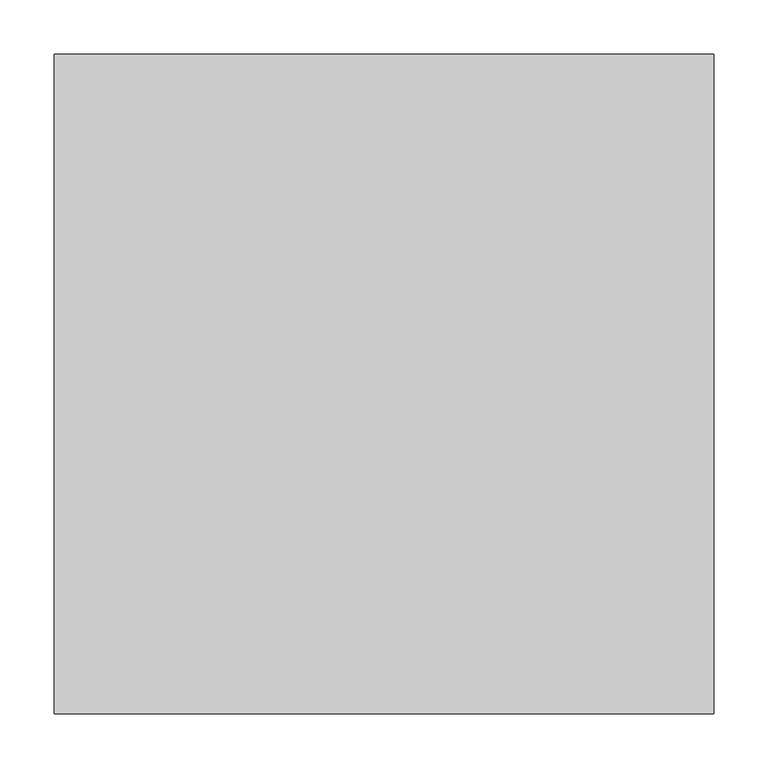
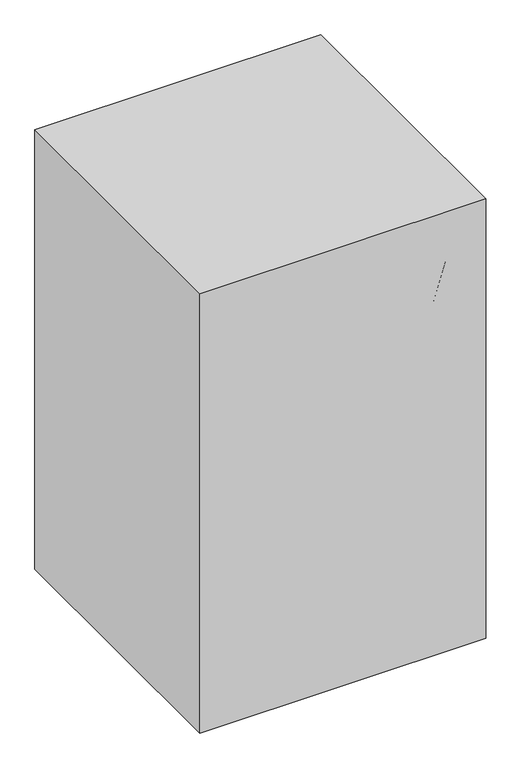
"""IFC4 building model written with IfcOpenShell, lengths in millimetres: proxy geometry, D3295 - Chair, Rotary, Laboratory, Dental : D3295 - Chair, Rotary, Laboratory, Dental."""

from ifc_helpers import new_model, si_unit, point, frame, frame_2d, origin, origin_with_axes, place, context, project, spatial, polyline, circle_curve, ellipse_curve, trimmed, segment, composite_curve, outline, extrude, source, transform, mapped, element, save
from ifc_brep_helpers import plane_surface, cylinder_surface, revolved_surface, advanced_brep


def specialty_equipment_802716e4(model_context):
    return source(origin(), model_context, "Body", "SolidModel", [
        advanced_brep(
        [(20.5891067, 39.0088165, 158.3164474), (12.606954, 21.8910347, 158.3164474), (12.606954, 21.8910347, 212.7487443), (20.5891067, 39.0088165, 212.7487443), (283.7284885, -83.6950923, 86.0096871), (283.7284885, -83.6950923, 57.6571213), (275.3053581, -100.6072429, 86.2220806), (287.501904, -95.8556376, 82.2734822), (275.3053581, -100.6072429, 57.8258095), (287.501904, -95.8556376, 54.689734)],
        [
            (0, 1),
            (1, 2),
            (2, 3),
            (3, 0),
            (3, 4),
            (4, 5),
            (5, 0),
            (2, 6),
            (6, 7, ellipse_curve(frame((278.918781, -91.8532617, 86.4074773), z_axis=(0.3625792018206629, -0.16907345849670724, 0.9164881276039822), x_axis=(0.8306203267741233, -0.3873246193939933, -0.40006188516396646)), 10.333389, 9.4704283)),
            (7, 4, ellipse_curve(frame((278.918781, -91.8532617, 86.4074773), z_axis=(0.3625792018206629, -0.16907345849670724, 0.9164881276039822), x_axis=(0.8306203267741233, -0.3873246193939933, -0.40006188516396646)), 10.333389, 9.4704283)),
            (1, 8),
            (8, 6),
            (5, 9, ellipse_curve(frame((278.918781, -91.8532617, 57.9730562), z_axis=(-0.2968743688836678, 0.13843479172039067, -0.9448287768380342), x_axis=(0.8563056778646188, -0.3993018953098915, -0.3275646233321667)), 10.0234334, 9.4704283)),
            (9, 8, ellipse_curve(frame((278.918781, -91.8532617, 57.9730562), z_axis=(-0.2968743688836678, 0.13843479172039067, -0.9448287768380342), x_axis=(0.8563056778646188, -0.3993018953098915, -0.3275646233321667)), 10.0234334, 9.4704283)),
            (9, 7),
        ],
        [
            plane_surface(frame((16.5980304, 30.4499256, 185.5325958), z_axis=(-0.9063077870366449, 0.42261826174071043, 0.0), x_axis=(-0.42261826174071043, -0.9063077870366449, 0.0))),
            plane_surface(frame((20.5891067, 39.0088165, 185.5325958), z_axis=(0.4226182617407104, 0.9063077870366448, 0.0), x_axis=(0.0, 0.0, 1.0))),
            plane_surface(frame((16.5980304, 30.4499256, 212.7487443), z_axis=(0.36257920182066294, -0.16907345849670727, 0.9164881276039825), x_axis=(-0.42261826174071043, -0.9063077870366449, 0.0))),
            plane_surface(frame((12.606954, 21.8910347, 185.5325958), z_axis=(-0.4226182617407102, -0.906307787036645, 0.0), x_axis=(0.0, 0.0, -1.0))),
            plane_surface(frame((16.5980304, 30.4499256, 158.3164474), z_axis=(-0.29687436888366786, 0.1384347917203907, -0.9448287768380345), x_axis=(0.42261826174071043, 0.9063077870366449, 0.0))),
            cylinder_surface(frame((278.918781, -91.8532617, 0.0), z_axis=(0.0, 0.0, -1.0000000000000002), x_axis=(-0.9063077870366449, 0.42261826174071043, 0.0)), 9.4704283),
        ],
        [
            (0, [[1, 2, 3, 4]]),
            (1, [[-4, 5, 6, 7]]),
            (2, [[-3, 8, 9, 10, -5]]),
            (3, [[-2, 11, 12, -8]]),
            (4, [[-1, -7, 13, 14, -11]]),
            (5, [[15, -9, -12, -14]]),
            (5, [[-15, -13, -6, -10]]),
        ],
    ),
        extrude(outline(composite_curve([segment(trimmed(circle_curve(frame_2d((-0.4565328, 38.3009494)), 25.4), [point((24.9434672, 38.3009494))], [point((-25.8565328, 38.3009494))], False, "CARTESIAN"), True, "CONTINUOUS"), segment(trimmed(circle_curve(frame_2d((-0.4565328, 38.3009494)), 25.4), [point((-25.8565328, 38.3009494))], [point((24.9434672, 38.3009494))], False, "CARTESIAN"), True, "CONTINUOUS")], self_intersect=False)), frame((0.0, 0.0, 154.0271692), z_axis=(0.0, 0.0, 1.0), x_axis=(1.0, 0.0, 0.0)), (0.0, 0.0, 1.0), 58.7215752),
        advanced_brep(
        [(-229.5082147, -153.1947504, 328.6387079), (232.0214447, -152.7605661, 328.5937403), (236.3508412, -177.6557493, 331.1720849), (-229.5082147, -178.826585, 331.293346), (-229.5082147, -246.1177228, 855.6310718), (-229.5082147, -269.2958289, 844.3699241), (236.3508412, -268.237077, 844.8843217), (232.0214447, -245.7251028, 855.8218273)],
        [
            (0, 1, circle_curve(frame((0.0, 1168.6045098, 191.7425871), z_axis=(0.0, 0.10301698777210262, 0.9946795967699159), x_axis=(-1.0, 0.0, 0.0)), 1348.5428628)),
            (1, 2, circle_curve(frame((232.0214447, -165.5806144, 329.9214872), z_axis=(0.0, -0.10301698777210262, -0.9946795967699159), x_axis=(-1.0, 0.0, 0.0)), 12.888621)),
            (2, 3, circle_curve(frame((0.0, 1168.6045098, 191.7425871), z_axis=(0.0, -0.10301698777210262, -0.9946795967699159), x_axis=(-1.0, 0.0, 0.0)), 1373.9428628)),
            (3, 0, circle_curve(frame((-229.5082147, -166.0106677, 329.9660269), z_axis=(0.0, -0.10301698777210262, -0.9946795967699159), x_axis=(-1.0, 0.0, 0.0)), 12.8844679)),
            (4, 5, circle_curve(frame((-229.5082147, -257.7067759, 850.0004979), z_axis=(0.0, -0.4370047614753844, 0.8994591922082082), x_axis=(-1.0, 0.0, 0.0)), 12.8844679)),
            (5, 6, circle_curve(frame((0.0, 949.1460573, 1436.3533187), z_axis=(0.0, -0.4370047614753844, 0.8994591922082082), x_axis=(-1.0, 0.0, 0.0)), 1373.9428628)),
            (6, 7, circle_curve(frame((232.0214447, -257.3178914, 850.1894385), z_axis=(0.0, -0.4370047614753844, 0.8994591922082082), x_axis=(-1.0, 0.0, 0.0)), 12.888621)),
            (7, 4, circle_curve(frame((0.0, 949.1460573, 1436.3533187), z_axis=(0.0, 0.4370047614753844, -0.8994591922082082), x_axis=(-1.0, 0.0, 0.0)), 1348.5428628)),
            (7, 1, circle_curve(frame((232.0214447, -1123.8751957, 429.1701512), z_axis=(-1.0, 0.0, 0.0), x_axis=(0.0, 0.9946795967699159, -0.10301698777210261)), 976.308987)),
            (0, 4, circle_curve(frame((-229.5082147, -1123.8751957, 429.1701512), z_axis=(1.0, 0.0, 0.0), x_axis=(0.0, 0.9946795967699159, -0.10301698777210261)), 975.8724803)),
            (6, 2, circle_curve(frame((236.3508412, -1123.8751957, 429.1701512), z_axis=(-1.0, 0.0, 0.0), x_axis=(0.0, 0.9946795967699159, -0.10301698777210261)), 951.280643)),
            (5, 3, circle_curve(frame((-229.5082147, -1123.8751957, 429.1701512), z_axis=(-1.0, 0.0, 0.0), x_axis=(0.0, 0.9946795967699159, -0.10301698777210261)), 950.1035446)),
        ],
        [
            plane_surface(frame((-317.5, -135.0564347, 326.7601586), z_axis=(0.0, -0.10301698777210258, -0.994679596769916), x_axis=(-1.0, 0.0, 0.0))),
            plane_surface(frame((-317.5, -229.715783, 863.6), z_axis=(0.0, -0.4370047614753844, 0.8994591922082082), x_axis=(-1.0, 0.0, 0.0))),
            revolved_surface(trimmed(ellipse_curve(frame((0.0, 1168.6045098, 191.7425871), z_axis=(0.0, 0.10301698777210262, 0.9946795967699159), x_axis=(-1.0, 0.0, 0.0)), 1348.5428628, 1348.5428628), [point((-229.5082147, -153.1947504, 328.6387079))], [point((232.0214447, -152.7605661, 328.5937403))], True, "CARTESIAN"), (-317.5, -1123.8751957, 429.1701512), (1.0, 0.0, 0.0)),
            revolved_surface(trimmed(ellipse_curve(frame((232.0214447, -165.5806144, 329.9214872), z_axis=(0.0, -0.10301698777210262, -0.9946795967699159), x_axis=(-1.0, 0.0, 0.0)), 12.888621, 12.888621), [point((232.0214447, -152.7605661, 328.5937403))], [point((236.3508412, -177.6557493, 331.1720849))], True, "CARTESIAN"), (-317.5, -1123.8751957, 429.1701512), (1.0, 0.0, 0.0)),
            revolved_surface(trimmed(ellipse_curve(frame((0.0, 1168.6045098, 191.7425871), z_axis=(0.0, -0.10301698777210262, -0.9946795967699159), x_axis=(-1.0, 0.0, 0.0)), 1373.9428628, 1373.9428628), [point((236.3508412, -177.6557493, 331.1720849))], [point((-229.5082147, -178.826585, 331.293346))], True, "CARTESIAN"), (-317.5, -1123.8751957, 429.1701512), (1.0, 0.0, 0.0)),
            revolved_surface(trimmed(ellipse_curve(frame((-229.5082147, -166.0106677, 329.9660269), z_axis=(0.0, -0.10301698777210262, -0.9946795967699159), x_axis=(-1.0, 0.0, 0.0)), 12.8844679, 12.8844679), [point((-229.5082147, -178.826585, 331.293346))], [point((-229.5082147, -153.1947504, 328.6387079))], True, "CARTESIAN"), (-317.5, -1123.8751957, 429.1701512), (1.0, 0.0, 0.0)),
        ],
        [
            (0, [[1, 2, 3, 4]]),
            (1, [[5, 6, 7, 8]]),
            (2, [[9, -1, 10, -8]]),
            (3, [[11, -2, -9, -7]]),
            (4, [[12, -3, -11, -6]]),
            (5, [[-10, -4, -12, -5]]),
        ],
    ),
        extrude(outline(composite_curve([segment(polyline([(-213.079753, -135.9379297), (-213.079753, 221.0075832)]), True, "CONTINUOUS"), segment(trimmed(circle_curve(frame_2d((-186.3342402, 221.0075832)), 26.7455128), [point((-213.079753, 221.0075832))], [point((-186.3342402, 247.753096))], False, "CARTESIAN"), True, "CONTINUOUS"), segment(polyline([(-186.3342402, 247.753096), (194.6657598, 247.753096)]), True, "CONTINUOUS"), segment(trimmed(circle_curve(frame_2d((194.6657598, 221.0075832)), 26.7455128), [point((194.6657598, 247.753096))], [point((221.4112726, 221.0075832))], False, "CARTESIAN"), True, "CONTINUOUS"), segment(polyline([(221.4112726, 221.0075832), (221.4112726, -135.9379297), (-213.079753, -135.9379297)]), True, "CONTINUOUS")], self_intersect=False)), frame((0.0, 0.0, 324.0440254), z_axis=(0.0, 0.0, 1.0), x_axis=(1.0, 0.0, 0.0)), (0.0, 0.0, 1.0), 67.8491407),
        advanced_brep(
        [(-213.079753, -134.5924168, 391.8931661), (-211.7342402, -135.9379297, 391.8931661), (-211.7342402, -135.9379297, 324.0440254), (-213.079753, -134.5924168, 324.0440254), (-213.079753, 221.0075832, 324.0440254), (-213.079753, 221.0075832, 391.8931661), (-186.3342402, 247.753096, 391.8931661), (-186.3342402, 247.753096, 324.0440254), (194.6657598, 247.753096, 324.0440254), (194.6657598, 247.753096, 391.8931661), (221.4112726, 221.0075832, 391.8931661), (221.4112726, 221.0075832, 324.0440254), (221.4112726, -134.5924168, 324.0440254), (221.4112726, -134.5924168, 391.8931661), (220.0657598, -135.9379297, 391.8931661), (220.0657598, -135.9379297, 324.0440254)],
        [
            (0, 1, circle_curve(frame((-211.7342402, -134.5924168, 391.8931661), z_axis=(0.0, 0.0, 1.0), x_axis=(0.0, -1.0, 0.0)), 1.3455128)),
            (1, 2),
            (2, 3, circle_curve(frame((-211.7342402, -134.5924168, 324.0440254), z_axis=(0.0, 0.0, -1.0), x_axis=(0.0, -1.0, 0.0)), 1.3455128)),
            (3, 0),
            (2, 1, circle_curve(frame((-211.7342402, -135.9379297, 357.9685958), z_axis=(-1.0, 0.0, 0.0), x_axis=(0.0, 1.0, 0.0)), 33.9245703)),
            (0, 3, circle_curve(frame((-213.079753, -134.5924168, 357.9685958), z_axis=(0.0, -1.0, 0.0), x_axis=(1.0, 0.0, 0.0)), 33.9245703)),
            (3, 4),
            (4, 5),
            (5, 0),
            (5, 4, circle_curve(frame((-213.079753, 221.0075832, 357.9685958), z_axis=(0.0, -1.0, 0.0), x_axis=(1.0, 0.0, 0.0)), 33.9245703)),
            (6, 5, circle_curve(frame((-186.3342402, 221.0075832, 391.8931661), z_axis=(0.0, 0.0, 1.0), x_axis=(-1.0, 0.0, 0.0)), 26.7455128)),
            (4, 7, circle_curve(frame((-186.3342402, 221.0075832, 324.0440254), z_axis=(0.0, 0.0, -1.0), x_axis=(-1.0, 0.0, 0.0)), 26.7455128)),
            (7, 6),
            (6, 7, circle_curve(frame((-186.3342402, 247.753096, 357.9685958), z_axis=(-1.0, 0.0, 0.0), x_axis=(0.0, -1.0, 0.0)), 33.9245703)),
            (7, 8),
            (8, 9),
            (9, 6),
            (9, 8, circle_curve(frame((194.6657598, 247.753096, 357.9685958), z_axis=(-1.0, 0.0, 0.0), x_axis=(0.0, -1.0, 0.0)), 33.9245703)),
            (10, 9, circle_curve(frame((194.6657598, 221.0075832, 391.8931661), z_axis=(0.0, 0.0, 1.0), x_axis=(0.0, 1.0, 0.0)), 26.7455128)),
            (8, 11, circle_curve(frame((194.6657598, 221.0075832, 324.0440254), z_axis=(0.0, 0.0, -1.0), x_axis=(0.0, 1.0, 0.0)), 26.7455128)),
            (11, 10),
            (10, 11, circle_curve(frame((221.4112726, 221.0075832, 357.9685958), z_axis=(0.0, 1.0, 0.0), x_axis=(-1.0, 0.0, 0.0)), 33.9245703)),
            (11, 12),
            (12, 13),
            (13, 10),
            (13, 12, circle_curve(frame((221.4112726, -134.5924168, 357.9685958), z_axis=(0.0, 1.0, 0.0), x_axis=(-1.0, 0.0, 0.0)), 33.9245703)),
            (14, 13, circle_curve(frame((220.0657598, -134.5924168, 391.8931661), z_axis=(0.0, 0.0, 1.0), x_axis=(1.0, 0.0, 0.0)), 1.3455128)),
            (12, 15, circle_curve(frame((220.0657598, -134.5924168, 324.0440254), z_axis=(0.0, 0.0, -1.0), x_axis=(1.0, 0.0, 0.0)), 1.3455128)),
            (15, 14),
            (14, 15, circle_curve(frame((220.0657598, -135.9379297, 357.9685958), z_axis=(1.0, 0.0, 0.0), x_axis=(0.0, 1.0, 0.0)), 33.9245703)),
            (15, 2),
            (1, 14),
        ],
        [
            revolved_surface(polyline([(-211.7342402, -135.9379296, 324.0440254), (-211.7342402, -135.9379296, 391.8931661)]), (-211.7342402, -134.5924168, 0.0), (0.0, 0.0, -1.0)),
            revolved_surface(trimmed(ellipse_curve(frame((-211.7342402, -135.9379297, 357.9685958), z_axis=(1.0, 0.0, 0.0), x_axis=(0.0, 1.0, 0.0)), 33.9245703, 33.9245703), [point((-211.7342402, -135.9379297, 391.8931661))], [point((-211.7342402, -135.9379297, 324.0440254))], True, "CARTESIAN"), (-211.7342402, -134.5924168, 0.0), (0.0, 0.0, -1.0)),
            plane_surface(frame((-213.079753, -134.5924168, 324.0440254), z_axis=(1.0, 0.0, 0.0), x_axis=(0.0, 1.0, 0.0))),
            cylinder_surface(frame((-213.079753, -134.5924168, 357.9685958), z_axis=(0.0, -1.0, 0.0), x_axis=(1.0, 0.0, 0.0)), 33.9245703),
            revolved_surface(polyline([(-213.079753, 221.0075832, 324.0440254), (-213.079753, 221.0075832, 391.8931661)]), (-186.3342402, 221.0075832, 0.0), (0.0, 0.0, -1.0)),
            revolved_surface(trimmed(ellipse_curve(frame((-213.079753, 221.0075832, 357.9685958), z_axis=(0.0, -1.0, 0.0), x_axis=(1.0, 0.0, 0.0)), 33.9245703, 33.9245703), [point((-213.079753, 221.0075832, 391.8931661))], [point((-213.079753, 221.0075832, 324.0440254))], True, "CARTESIAN"), (-186.3342402, 221.0075832, 0.0), (0.0, 0.0, -1.0)),
            plane_surface(frame((-186.3342402, 247.753096, 324.0440254), z_axis=(0.0, -1.0, 0.0), x_axis=(1.0, 0.0, 0.0))),
            cylinder_surface(frame((-186.3342402, 247.753096, 357.9685958), z_axis=(-1.0, 0.0, 0.0), x_axis=(0.0, -1.0, 0.0)), 33.9245703),
            revolved_surface(polyline([(194.6657598, 247.753096, 324.0440254), (194.6657598, 247.753096, 391.8931661)]), (194.6657598, 221.0075832, 0.0), (0.0, 0.0, -1.0)),
            revolved_surface(trimmed(ellipse_curve(frame((194.6657598, 247.753096, 357.9685958), z_axis=(-1.0, 0.0, 0.0), x_axis=(0.0, -1.0, 0.0)), 33.9245703, 33.9245703), [point((194.6657598, 247.753096, 391.8931661))], [point((194.6657598, 247.753096, 324.0440254))], True, "CARTESIAN"), (194.6657598, 221.0075832, 0.0), (0.0, 0.0, -1.0)),
            plane_surface(frame((221.4112726, 221.0075832, 324.0440254), z_axis=(-1.0, 0.0, 0.0), x_axis=(0.0, -1.0, 0.0))),
            cylinder_surface(frame((221.4112726, 221.0075832, 357.9685958), z_axis=(0.0, 1.0, 0.0), x_axis=(-1.0, 0.0, 0.0)), 33.9245703),
            revolved_surface(polyline([(221.4112726, -134.5924168, 324.0440254), (221.4112726, -134.5924168, 391.8931661)]), (220.0657598, -134.5924168, 0.0), (0.0, 0.0, -1.0)),
            revolved_surface(trimmed(ellipse_curve(frame((221.4112726, -134.5924168, 357.9685958), z_axis=(0.0, 1.0, 0.0), x_axis=(-1.0, 0.0, 0.0)), 33.9245703, 33.9245703), [point((221.4112726, -134.5924168, 391.8931661))], [point((221.4112726, -134.5924168, 324.0440254))], True, "CARTESIAN"), (220.0657598, -134.5924168, 0.0), (0.0, 0.0, -1.0)),
            plane_surface(frame((220.0657598, -135.9379297, 324.0440254), z_axis=(0.0, 1.0, 0.0), x_axis=(-1.0, 0.0, 0.0))),
            cylinder_surface(frame((220.0657598, -135.9379297, 357.9685958), z_axis=(1.0, 0.0, 0.0), x_axis=(0.0, 1.0, 0.0)), 33.9245703),
        ],
        [
            (0, [[1, 2, 3, 4]]),
            (1, [[-3, 5, -1, 6]]),
            (2, [[-4, 7, 8, 9]]),
            (3, [[-6, -9, 10, -7]]),
            (4, [[11, -8, 12, 13]]),
            (5, [[-12, -10, -11, 14]]),
            (6, [[-13, 15, 16, 17]]),
            (7, [[-14, -17, 18, -15]]),
            (8, [[19, -16, 20, 21]]),
            (9, [[-20, -18, -19, 22]]),
            (10, [[-21, 23, 24, 25]]),
            (11, [[-22, -25, 26, -23]]),
            (12, [[27, -24, 28, 29]]),
            (13, [[-28, -26, -27, 30]]),
            (14, [[-29, 31, -2, 32]]),
            (15, [[-30, -32, -5, -31]]),
        ],
    ),
        extrude(outline(composite_curve([segment(trimmed(circle_curve(frame_2d((0.0, 38.1)), 12.7), [point((12.7, 38.1))], [point((-12.7, 38.1))], False, "CARTESIAN"), True, "CONTINUOUS"), segment(trimmed(circle_curve(frame_2d((0.0, 38.1)), 12.7), [point((-12.7, 38.1))], [point((12.7, 38.1))], False, "CARTESIAN"), True, "CONTINUOUS")], self_intersect=False)), frame((0.0, 0.0, 212.7487443), z_axis=(0.0, 0.0, 1.0), x_axis=(1.0, 0.0, 0.0)), (0.0, 0.0, 1.0), 66.217703),
        extrude(outline(polyline([(304.8, 304.8), (304.8, -304.8), (-304.8, -304.8), (-304.8, 304.8), (304.8, 304.8)])), origin_with_axes(), (0.0, 0.0, 1.0), 990.6),
    ])


if __name__ == "__main__":
    model = new_model("IFC4")
    model_context = context("Model", 3, world=origin())
    ifc_project = project(units=[si_unit("LENGTHUNIT", "METRE", prefix="MILLI")], contexts=[model_context])
    site = spatial("IfcSite", under=ifc_project)
    building = spatial("IfcBuilding", under=site)
    placement = place(None, origin())
    specialty_equipment_shape = specialty_equipment_802716e4(model_context)
    element("IfcBuildingElementProxy", 1, Name="D3295 - Chair, Rotary, Laboratory, Dental : D3295 - Chair, Rotary, Laboratory, Dental", ObjectType="D3295 - Chair, Rotary, Laboratory, Dental : D3295 - Chair, Rotary, Laboratory, Dental", at=placement, inside=building, context=model_context, shape_type="MappedRepresentation", body=[
        mapped(specialty_equipment_shape, transform((0.0, 0.0, 0.0), x_axis=(1.0, 0.0, 0.0), y_axis=(0.0, 1.0, 0.0), z_axis=(0.0, 0.0, 1.0))),
    ])
    save(model, "model.ifc")

# Revit data of these elements
# Type "D3295 - Chair, Rotary, Laboratory, Dental : D3295 - Chair, Rotary, Laboratory, Dental"
#   Watts2 = "0"
#   Watts1 = "0"
#   Unit_Issue = "EA"
#   UTIL_6_Misc = "-"
#   UTIL_5_NonMedGas = "-"
#   UTIL_4_MiscGas = "-"
#   UTIL_3_MedGas = "-"
#   UTIL_2_Elec = "-"
#   UTIL_1_WaterDrain = "-"
#   Nomenclature = "Chair, Rotary, Laboratory, Dental"
#   NSN = "6520"
#   Location [instance default] = ""
#   JSN = "D3295"
#   Fund_Source_VA = "-"
#   Fund_Source_Navy = "-"
#   Fund_Source_Army = "-"
#   Fund_Source_AF = "-"
#   ELEC_Volts2 = "0"
#   ELEC_Volts1 = "0"
#   ELEC_Phase2 = "0"
#   ELEC_Phase1 = "0"
#   ELEC_HertzSwitch = "0"
#   ELEC_HertzDependent = "0"
#   ELEC_Hertz = "0"
#   ELEC_Amps2 = "0"
#   ELEC_Amps1 = "0"
#   DetailDescription = "Rotary dental laboratory chair. The chair is used by technicians while working at a bench. Chairs also have casters and an adjustable backrest."
#   CAT_VA = "C"
#   CAT_Navy = "C"
#   CAT_IHS = "-"
#   CAT_Army = "C"
#   CAT_AF = "C"
#   BTUperhour = "0"
#   Weight_IP = 36
#   DIM_Width_IP = 2' - 0"
#   DIM_Height_IP = 3' - 0"
#   DIM_Depth_IP = 2' - 0"
#   Assembly Code = ""
# Element 1 (IfcBuildingElementProxy, "D3295 - Chair, Rotary, Laboratory, Dental : D3295 - Chair, Rotary, Laboratory, Dental")
#   Location = "DNPL2"
#   Materials on its faces: "00 - bernhardt blitz - base", "00 - bernhardt blitz - Seat Fabric", "00 - bernhardt blitz - wheels", "00 - bernhardt blitz - arms", "00 - bernhardt blitz - mechanic", "00 - bernhardt blitz - Back Fabric", "EquipSpace"
# Materials
#   "00 - bernhardt blitz - base": class "Miscellaneous", colour RGB 192 192 192, transparency 0
#   "00 - bernhardt blitz - Seat Fabric": class "Miscellaneous", colour RGB 188 173 117, transparency 0
#   "00 - bernhardt blitz - wheels": class "Miscellaneous", colour RGB 51 51 51, transparency 0
#   "00 - bernhardt blitz - arms": class "Miscellaneous", colour RGB 51 51 51, transparency 0
#   "00 - bernhardt blitz - mechanic": class "Miscellaneous", colour RGB 62 62 62, transparency 0
#   "00 - bernhardt blitz - Back Fabric": class "Miscellaneous", colour RGB 93 93 93, transparency 0
#   "EquipSpace": class "Unassigned", colour RGB 221 217 195, transparency 0.5
